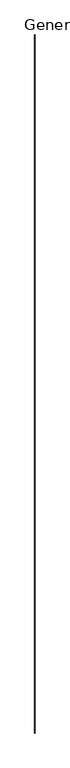
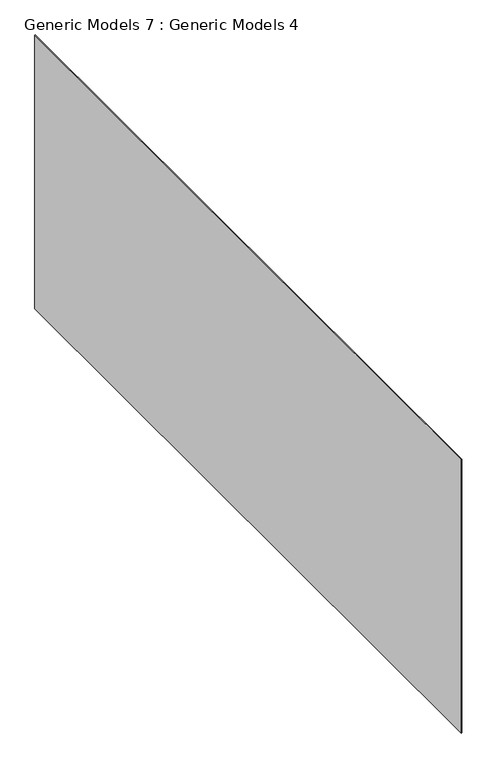
"""IFC4 building model written with IfcOpenShell, lengths in millimetres: proxy geometry, Generic Models 7 : Generic Models 4."""

from ifc_helpers import new_model, si_unit, frame, origin, place, context, project, spatial, polyline, outline, extrude, source, transform, mapped, element, save


def generic_models_7_generic_models_4_32dcae1e(model_context):
    return source(origin(), model_context, "Body", "SweptSolid", [
        extrude(outline(polyline([(594556.5576893, -527524.3545647), (594556.5576893, -584979.050959), (594531.1576893, -584979.050959), (594531.1576893, -527524.3545647), (594556.5576893, -527524.3545647)])), frame((0.0, 0.0, -2503.337634), z_axis=(0.0, 0.0, 1.0), x_axis=(1.0, 0.0, 0.0)), (0.0, 0.0, 1.0), 22488.6259865),
    ])


if __name__ == "__main__":
    model = new_model("IFC4")
    model_context = context("Model", 3, world=origin())
    ifc_project = project(units=[si_unit("LENGTHUNIT", "METRE", prefix="MILLI")], contexts=[model_context])
    site = spatial("IfcSite", under=ifc_project)
    building = spatial("IfcBuilding", under=site)
    placement = place(None, origin())
    generic_models_7_generic_models_4_shape = generic_models_7_generic_models_4_32dcae1e(model_context)
    element("IfcBuildingElementProxy", 1, Name="Generic Models 7 : Generic Models 4", ObjectType="Generic Models 7 : Generic Models 4", at=placement, inside=building, context=model_context, shape_type="MappedRepresentation", body=[
        mapped(generic_models_7_generic_models_4_shape, transform((0.0, 0.0, 0.0), x_axis=(1.0, 0.0, 0.0), y_axis=(0.0, 1.0, 0.0), z_axis=(0.0, 0.0, 1.0))),
    ])
    save(model, "model.ifc")

# Revit data of these elements
# Element 1 (IfcBuildingElementProxy, "Generic Models 7 : Generic Models 4")
#   Materials on its faces: "Air"
# Materials
#   "Air": class "Gas", colour RGB 255 255 255, transparency 1, Description = "Air", Cost = 0
